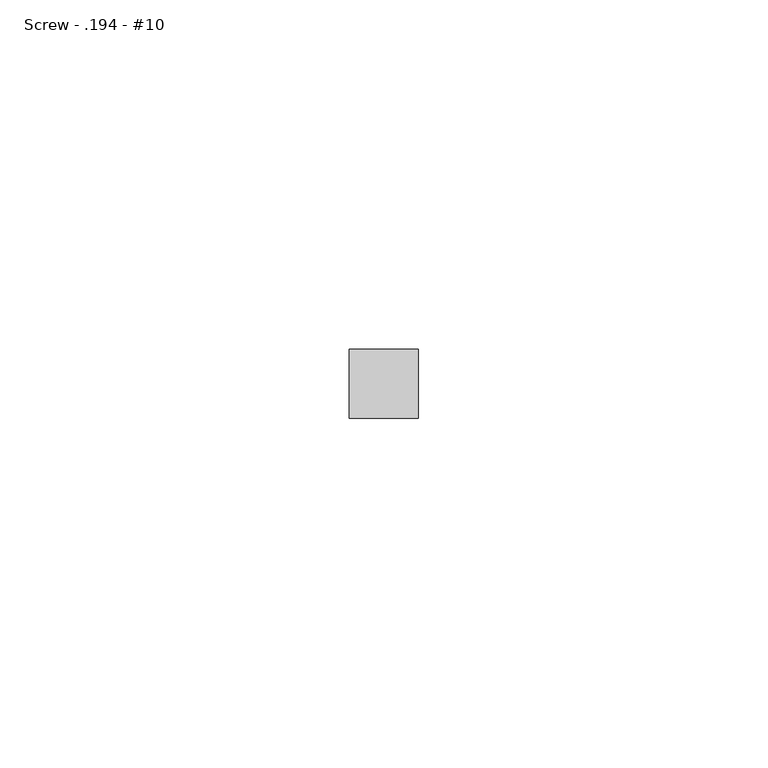
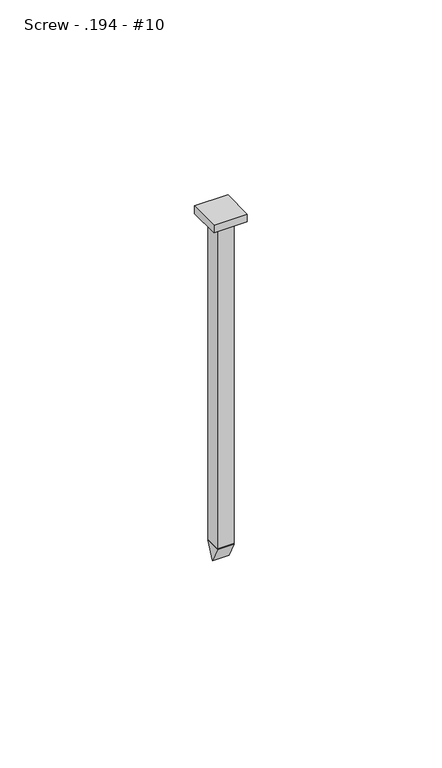
"""IFC4 building model written with IfcOpenShell, lengths in millimetres: fastener geometry, 060523 - W_P_C - Fastenings - Generic - SQUARE : Screw - .194 - #10."""

from ifc_helpers import new_model, si_unit, frame, origin, origin_with_axes, place, context, project, spatial, polyline, outline, extrude, source, transform, mapped, element, save


def screw_194_10_41c9de8e(model_context):
    return source(origin(), model_context, "Body", "SweptSolid", [
        extrude(outline(polyline([(0.0, -106.5276), (-2.4638, -101.6), (2.4638, -101.6), (0.0, -106.5276)])), frame((-2.4638, 0.0, 0.0), z_axis=(1.0, 0.0, 0.0), x_axis=(0.0, 1.0, 0.0)), (0.0, 0.0, 1.0), 4.9276),
        extrude(outline(polyline([(-4.9276, -4.9276), (-4.9276, 4.9276), (4.9276, 4.9276), (4.9276, -4.9276), (-4.9276, -4.9276)])), origin_with_axes(), (0.0, 0.0, 1.0), 2.4638),
        extrude(outline(polyline([(-2.4638, 2.4638), (2.4638, 2.4638), (2.4638, -2.4638), (-2.4638, -2.4638), (-2.4638, 2.4638)])), frame((0.0, 0.0, -101.6), z_axis=(0.0, 0.0, 1.0), x_axis=(1.0, 0.0, 0.0)), (0.0, 0.0, 1.0), 101.6),
    ])


if __name__ == "__main__":
    model = new_model("IFC4")
    model_context = context("Model", 3, world=origin())
    ifc_project = project(units=[si_unit("LENGTHUNIT", "METRE", prefix="MILLI")], contexts=[model_context])
    site = spatial("IfcSite", under=ifc_project)
    building = spatial("IfcBuilding", under=site)
    placement = place(None, origin())
    screw_194_10_shape = screw_194_10_41c9de8e(model_context)
    element("IfcFastener", 1, ObjectType="060523 - W_P_C - Fastenings - Generic - SQUARE : Screw - .194 - #10", at=placement, inside=building, context=model_context, shape_type="MappedRepresentation", body=[
        mapped(screw_194_10_shape, transform((0.0, 0.0, 0.0), x_axis=(1.0, 0.0, 0.0), y_axis=(0.0, 1.0, 0.0), z_axis=(0.0, 0.0, 1.0))),
    ])
    save(model, "model.ifc")

# Revit data of these elements
# Type "060523 - W_P_C - Fastenings - Generic - SQUARE : Screw - .194 - #10"
#   Washer_Thickness = 0' - 0.00333"
#   Washer Radius = 0' - 0.107"
#   Washer Offset - Head = 0' - 0"
#   Washer Offset = 0' - 0"
#   Thickness_of_Substrate [instance default] = 0' - 1"
#   Side = 0' - 0 37/64"
#   Radius = 0' - 0.097"
#   Length [instance default] = 0' - 4"
#   Head Size = 0' - 1"
#   Head Radius = 0' - 0 1/2"
#   Head Height = 0' - 0.01"
#   Double Diameter = 0' - 0.388"
#   Diameter = 0' - 0.194"
#   Default Elevation = 4' - 0"
#   Washer_Nut_Visibility = no
#   Washer_Head_Visibility = no
#   Round_Head_Visibility = yes
#   Point Visibility = yes
#   Nut_Visibility = no
#   Hex_Head_Visiblilty = no
#   Washer Material = none
#   Bolt Material (Size) = AT SILL - FASTENER AT 24" O.C.
# Materials
#   "AT SILL - FASTENER AT 24\" O.C.": class "Generic", colour RGB 120 120 120, transparency 0, Cost = 0
